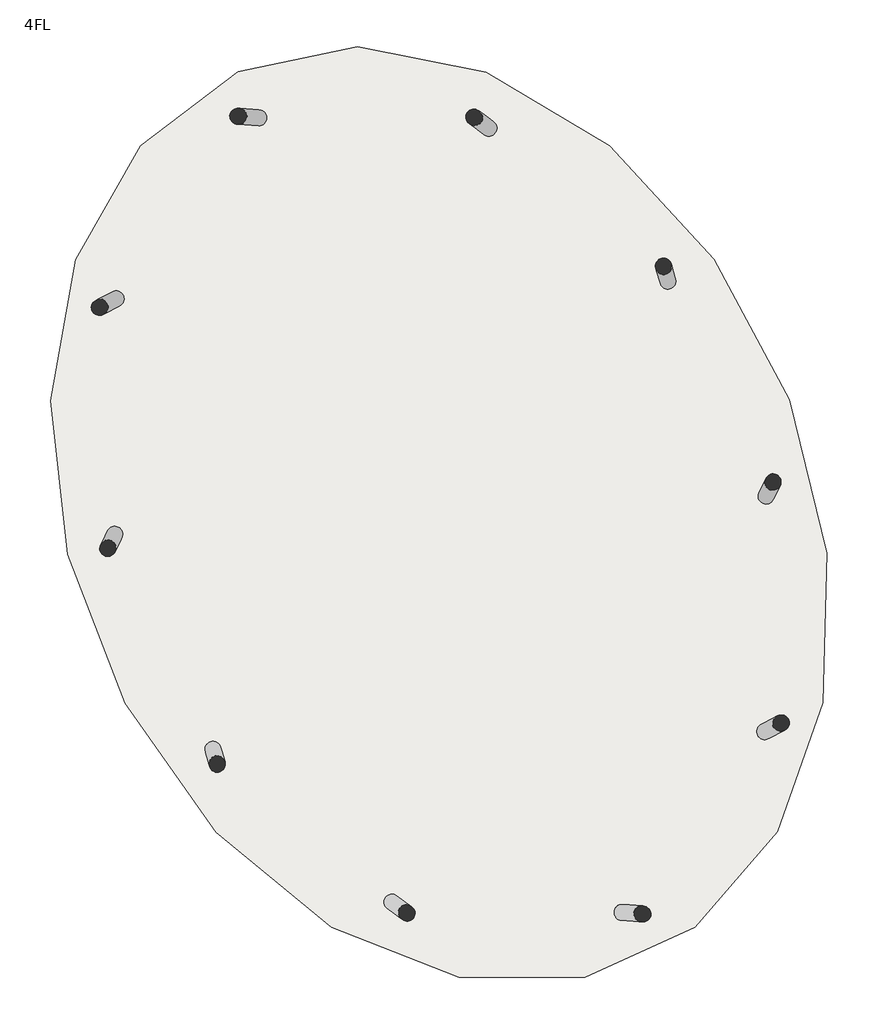
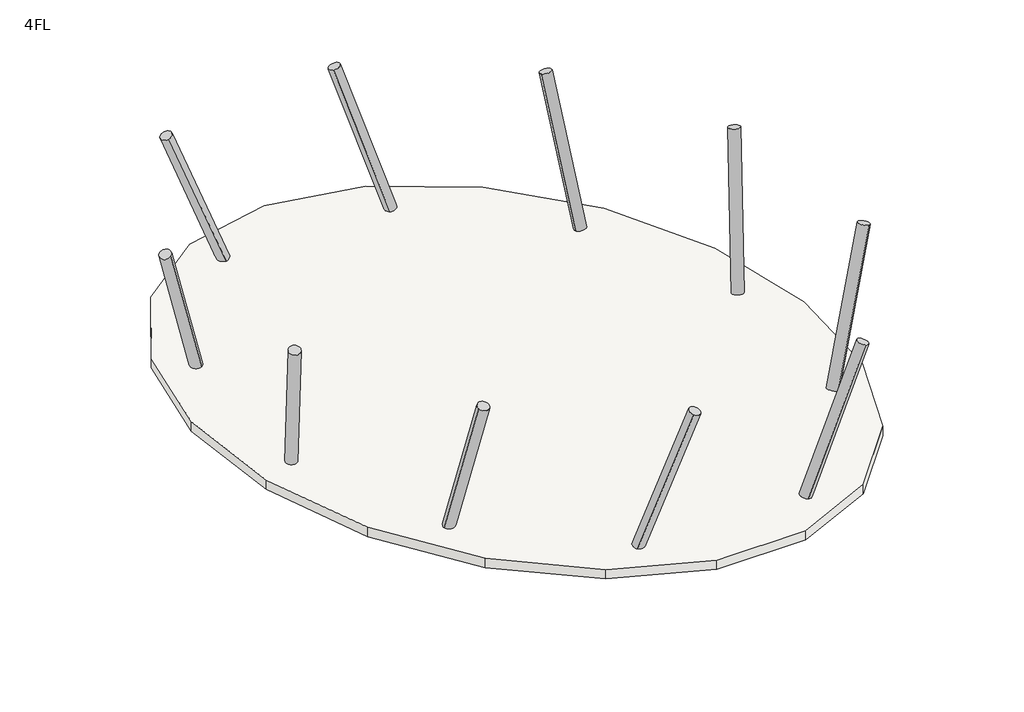
# One storey: 10 columns, 1 slab.
"""IFC4 building model written with IfcOpenShell, lengths in millimetres."""

from ifc_helpers import new_model, si_unit, point, frame, frame_2d, origin, place, context, project, spatial, polyline, circle_curve, trimmed, segment, composite_curve, outline, extrude, element, save

model = new_model("IFC4")

# Units and contexts
model_context = context("Model", 3, world=origin())
ifc_project = project(units=[si_unit("LENGTHUNIT", "METRE", prefix="MILLI")], contexts=[model_context])

# Site, building, storey
site = spatial("IfcSite", under=ifc_project)
building = spatial("IfcBuilding", under=site)
storey = spatial("IfcBuildingStorey", under=building, Name="4FL", Elevation=13500.0)

# Columns
placement = place(None, origin())
element("IfcColumn", 1, ObjectType="コンクリート-円形-柱 : 750", at=placement, inside=storey, context=model_context, shape_type="SweptSolid", body=[
    extrude(outline(composite_curve([segment(trimmed(circle_curve(frame_2d((0.0, -175.0000001)), 175.0), [point((0.0, -350.0))], [point((0.0, 0.0))], False, "CARTESIAN"), True, "CONTINUOUS"), segment(trimmed(circle_curve(frame_2d((0.0, -175.0000001)), 175.0), [point((0.0, 0.0))], [point((0.0, -350.0))], False, "CARTESIAN"), True, "CONTINUOUS")], self_intersect=False)), frame((-3973.6346017, 8498.3571824, 13500.0), z_axis=(-0.3520323783253696, 0.025941957714595305, 0.9356282485263674), x_axis=(-0.93309808166636, 0.06876183120799671, -0.3529869410608302)), (0.0, 0.0, 1.0), 4809.6025393),
])
element("IfcColumn", 2, ObjectType="コンクリート-円形-柱 : 750", at=placement, inside=storey, context=model_context, shape_type="SweptSolid", body=[
    extrude(outline(composite_curve([segment(trimmed(circle_curve(frame_2d((0.0, -175.0)), 175.0), [point((0.0, -350.0))], [point((0.0, 0.0))], False, "CARTESIAN"), True, "CONTINUOUS"), segment(trimmed(circle_curve(frame_2d((0.0, -175.0)), 175.0), [point((0.0, 0.0))], [point((0.0, -350.0))], False, "CARTESIAN"), True, "CONTINUOUS")], self_intersect=False)), frame((-6998.049403, 4571.3361205, 13500.0), z_axis=(-0.2857036103414105, -0.14758179057693752, 0.9468859815880624), x_axis=(-0.8412761492031519, -0.43456587867653, -0.3215694915131278)), (0.0, 0.0, 1.0), 4752.4201303),
])
element("IfcColumn", 3, ObjectType="コンクリート-円形-柱 : 750", at=placement, inside=storey, context=model_context, shape_type="SweptSolid", body=[
    extrude(outline(composite_curve([segment(trimmed(circle_curve(frame_2d((0.0, -175.0000001)), 175.0), [point((0.0, -350.0))], [point((0.0, 0.0))], False, "CARTESIAN"), True, "CONTINUOUS"), segment(trimmed(circle_curve(frame_2d((0.0, -175.0000001)), 175.0), [point((0.0, 0.0))], [point((0.0, -350.0))], False, "CARTESIAN"), True, "CONTINUOUS")], self_intersect=False)), frame((-6955.2646915, -489.9218359, 13500.0), z_axis=(-0.1209332009873062, -0.2467821925563094, 0.9614955591868662), x_axis=(-0.423100711999237, -0.8633999640038232, -0.2748204680585774)), (0.0, 0.0, 1.0), 4680.2088236),
])
element("IfcColumn", 4, ObjectType="コンクリート-円形-柱 : 750", at=placement, inside=storey, context=model_context, shape_type="SweptSolid", body=[
    extrude(outline(composite_curve([segment(trimmed(circle_curve(frame_2d((0.0, -175.0000001)), 175.0), [point((0.0, -350.0000001))], [point((0.0, 0.0))], False, "CARTESIAN"), True, "CONTINUOUS"), segment(trimmed(circle_curve(frame_2d((0.0, -175.0000001)), 175.0), [point((0.0, 0.0))], [point((0.0, -350.0000001))], False, "CARTESIAN"), True, "CONTINUOUS")], self_intersect=False)), frame((-4801.5324839, -5056.3710466, 13500.0), z_axis=(0.075620596245678, -0.2625861836338081, 0.9619407578370303), x_axis=(0.2662045111309179, -0.9243728575859578, -0.27325808023171033)), (0.0, 0.0, 1.0), 4678.0427623),
])
element("IfcColumn", 5, ObjectType="コンクリート-円形-柱 : 750", at=placement, inside=storey, context=model_context, shape_type="SweptSolid", body=[
    extrude(outline(composite_curve([segment(trimmed(circle_curve(frame_2d((0.0, -174.9999999)), 175.0), [point((0.0, -350.0))], [point((0.0, 0.0))], False, "CARTESIAN"), True, "CONTINUOUS"), segment(trimmed(circle_curve(frame_2d((0.0, -174.9999999)), 175.0), [point((0.0, 0.0))], [point((0.0, -350.0))], False, "CARTESIAN"), True, "CONTINUOUS")], self_intersect=False)), frame((-959.0907842, -8304.1052281, 13500.0), z_axis=(0.2569549892747412, -0.18976265971306566, 0.9476097648639132), x_axis=(0.7622728235591315, -0.5629426337813029, -0.3194303265730402)), (0.0, 0.0, 1.0), 4748.7902371),
])
element("IfcColumn", 6, ObjectType="コンクリート-円形-柱 : 750", at=placement, inside=storey, context=model_context, shape_type="SweptSolid", body=[
    extrude(outline(composite_curve([segment(trimmed(circle_curve(frame_2d((0.0, -175.0)), 175.0), [point((0.0, -350.0))], [point((0.0, 0.0))], False, "CARTESIAN"), True, "CONTINUOUS"), segment(trimmed(circle_curve(frame_2d((0.0, -175.0)), 175.0), [point((0.0, 0.0))], [point((0.0, -350.0))], False, "CARTESIAN"), True, "CONTINUOUS")], self_intersect=False)), frame((3973.6346381, -8498.3571826, 13500.0), z_axis=(0.3520323784242424, -0.025941956908569826, 0.9356282485115148), x_axis=(0.9330980818095522, -0.06876182906278264, -0.3529869411001986)), (0.0, 0.0, 1.0), 4809.6025393),
])
element("IfcColumn", 7, ObjectType="コンクリート-円形-柱 : 750", at=placement, inside=storey, context=model_context, shape_type="SweptSolid", body=[
    extrude(outline(composite_curve([segment(trimmed(circle_curve(frame_2d((0.0, -175.0)), 175.0), [point((0.0, -349.9999999))], [point((0.0, 0.0))], False, "CARTESIAN"), True, "CONTINUOUS"), segment(trimmed(circle_curve(frame_2d((0.0, -175.0)), 175.0), [point((0.0, 0.0))], [point((0.0, -349.9999999))], False, "CARTESIAN"), True, "CONTINUOUS")], self_intersect=False)), frame((6998.049395, -4571.3360767, 13500.0), z_axis=(0.2857036111394765, 0.1475817868621404, 0.9468859819262511), x_axis=(0.8412761544588145, 0.43456586923897916, -0.3215694905173055)), (0.0, 0.0, 1.0), 4752.4201303),
])
element("IfcColumn", 8, ObjectType="コンクリート-円形-柱 : 750", at=placement, inside=storey, context=model_context, shape_type="SweptSolid", body=[
    extrude(outline(composite_curve([segment(trimmed(circle_curve(frame_2d((-1e-07, -175.0)), 175.0), [point((-1e-07, -350.0))], [point((0.0, 0.0))], False, "CARTESIAN"), True, "CONTINUOUS"), segment(trimmed(circle_curve(frame_2d((-1e-07, -175.0)), 175.0), [point((0.0, 0.0))], [point((-1e-07, -350.0))], False, "CARTESIAN"), True, "CONTINUOUS")], self_intersect=False)), frame((6955.2646666, 489.9218707, 13500.0), z_axis=(0.12093320165250103, 0.2467821890780112, 0.9614955599959577), x_axis=(0.4231007190405781, 0.8633999614542996, -0.27482046522786424)), (0.0, 0.0, 1.0), 4680.2088236),
])
element("IfcColumn", 9, ObjectType="コンクリート-円形-柱 : 750", at=placement, inside=storey, context=model_context, shape_type="SweptSolid", body=[
    extrude(outline(composite_curve([segment(trimmed(circle_curve(frame_2d((0.0, -175.0)), 175.0), [point((0.0, -350.0))], [point((0.0, 0.0))], False, "CARTESIAN"), True, "CONTINUOUS"), segment(trimmed(circle_curve(frame_2d((0.0, -175.0)), 175.0), [point((0.0, 0.0))], [point((0.0, -350.0))], False, "CARTESIAN"), True, "CONTINUOUS")], self_intersect=False)), frame((4801.5324879, 5056.3710446, 13500.0), z_axis=(-0.075620590968162, 0.2625861792891104, 0.961940759437905), x_axis=(-0.26620449848571953, 0.9243728628935078, -0.27325807459620816)), (0.0, 0.0, 1.0), 4678.0427518),
])
element("IfcColumn", 10, ObjectType="コンクリート-円形-柱 : 750", at=placement, inside=storey, context=model_context, shape_type="SweptSolid", body=[
    extrude(outline(composite_curve([segment(trimmed(circle_curve(frame_2d((0.0, -175.0000001)), 175.0), [point((0.0, -350.0))], [point((0.0, 0.0))], False, "CARTESIAN"), True, "CONTINUOUS"), segment(trimmed(circle_curve(frame_2d((0.0, -175.0000001)), 175.0), [point((0.0, 0.0))], [point((0.0, -350.0))], False, "CARTESIAN"), True, "CONTINUOUS")], self_intersect=False)), frame((959.0908118, 8304.1052391, 13500.0), z_axis=(-0.2569549800273546, 0.18976265602019352, 0.9476097681109579), x_axis=(-0.7622728217248291, 0.5629426417309054, -0.31943031694048163)), (0.0, 0.0, 1.0), 4748.7902217),
])

# Slab
element("IfcSlab", 11, ObjectType="一般 300 mm", at=placement, inside=storey, context=model_context, shape_type="SweptSolid", body=[
    extrude(outline(polyline([(-7963.1456311, 5580.4907716), (-6549.3830561, 8064.952189), (-4418.7457038, 9675.7034427), (-1806.150389, 10231.1139666), (997.2978672, 9672.5882037), (3686.7082807, 8067.313984), (5974.8340174, 5592.5233247), (7617.8472272, 2515.6435883), (8439.783936, -832.8046707), (8351.012355, -4093.7163525), (7357.3555117, -6916.5286454), (5560.7962734, -8993.5077187), (3155.2924954, -10092.0644627), (409.1203506, -10089.6813333), (-2374.9256895, -8992.0881298), (-4897.4913401, -6923.734213), (-6889.8255945, -4109.7885902), (-8139.2313168, -853.1543372), (-8511.1496, 2496.7389427), (-7963.1456311, 5580.4907716)])), frame((0.0, 0.0, 13200.0), z_axis=(0.0, 0.0, 1.0), x_axis=(1.0, 0.0, 0.0)), (0.0, 0.0, 1.0), 300.0),
])

save(model, "model.ifc")

# Revit data of these elements
# Type "コンクリート-円形-柱 : 750"
#   Keynote = "03310.Q1"
#   R = 350 mm
#   Structural Material [instance default] = コンクリート - 現場打ち
# Type "一般 300 mm"
#   Function = 0
#   Layers, outside or top first: 300 mm no material (function 1)
# Elements 1, 2, 3, 4, 5, 6, 7, 8, 9, 10 (IfcColumn, "コンクリート-円形-柱 : 750")
#   Structural Material = コンクリート - 現場打ち
#   Phase Created = 新しい建設
#   Materials on its faces: "コンクリート - 現場打ち"
# Element 11 (IfcSlab, "一般 300 mm")
#   Height Offset From Level = 0 mm
#   Phase Created = 新しい建設
# Materials
#   "コンクリート - 現場打ち": class "コンクリート", colour RGB 192 192 192, transparency 0
